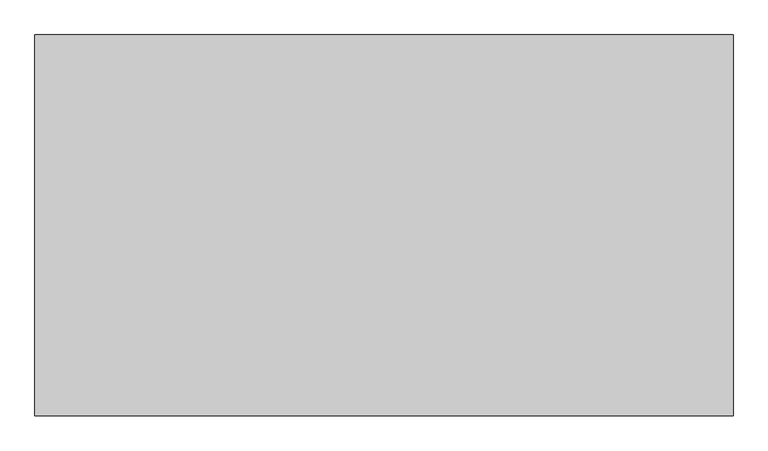
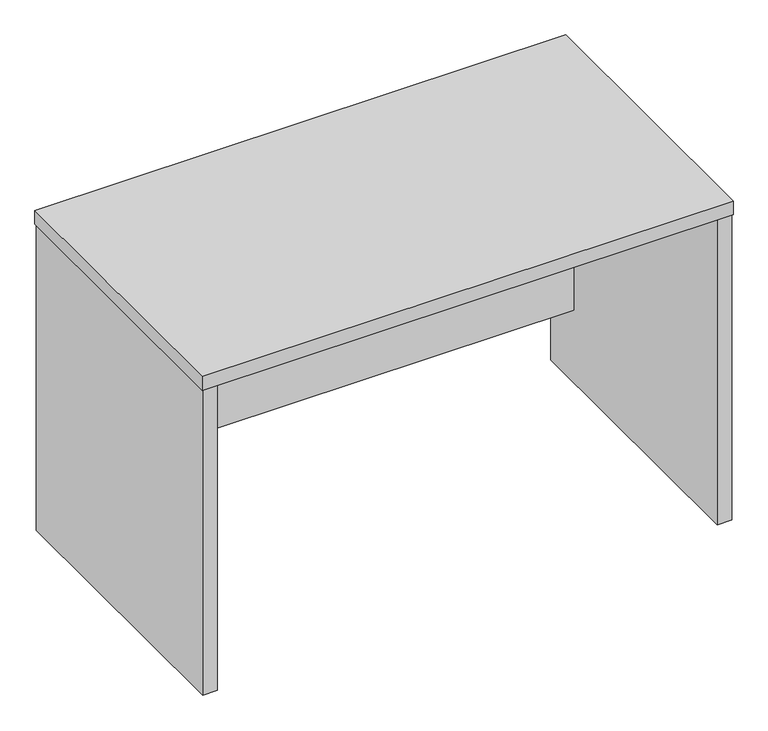
"""IFC4 building model written with IfcOpenShell, lengths in millimetres: furniture geometry, GEL-Table-一般オフィスデスク : GEL-Table-一般オフィスデスク."""

import ifcopenshell
import ifcopenshell.guid

model = None  # the IFC model being written
_history = None  # IfcOwnerHistory: only IFC2X3 demands one
_inside = {}  # id of a spatial element -> (the spatial element, [elements in it])
_under = {}  # id of a project, library or spatial element -> (it, [spatial elements below it])
_declared = {}  # id of a project -> (the project, [libraries it declares])
_typed = {}  # id of a type object -> (the type object, [elements of that type])
_made_of = {}  # id of a material, layer set ... -> (it, [elements and type objects made of it])


def new_model(schema):
    """Start an empty IFC model of exactly this schema.

    Asked for "IFC4X3", IfcOpenShell would pick the latest addendum, in which some entities
    have other attributes; the version numbers below select the first issue.
    IFC2X3 requires an IfcOwnerHistory on every rooted entity: one is made here for all.
    """
    global model, _history
    if schema == "IFC4X3":
        model = ifcopenshell.file(schema_version=(4, 3, 0, 0))
    else:
        model = ifcopenshell.file(schema=schema)
    _inside.clear()
    _under.clear()
    _declared.clear()
    _typed.clear()
    _made_of.clear()
    _history = None
    if model.schema == "IFC2X3":
        org = make("IfcOrganization", Name="unknown")
        user = make(
            "IfcPersonAndOrganization",
            ThePerson=make("IfcPerson", FamilyName="unknown"),
            TheOrganization=org,
        )
        app = make(
            "IfcApplication",
            ApplicationDeveloper=org,
            Version="unknown",
            ApplicationFullName="unknown",
            ApplicationIdentifier="unknown",
        )
        _history = make(
            "IfcOwnerHistory",
            OwningUser=user,
            OwningApplication=app,
            ChangeAction="ADDED",
            CreationDate=0,
        )
    return model


def make(cls, **values):
    """One entity of the class cls with the attributes given. An attribute that is None is left unset."""
    return model.create_entity(
        cls, **{name: value for name, value in values.items() if value is not None}
    )


def rooted(cls, **values):
    """An entity with a GlobalId (a new one), such as an element, a storey or a relation."""
    return make(cls, GlobalId=ifcopenshell.guid.new(), OwnerHistory=_history, **values)


def si_unit(unit_type, name, prefix=None):
    """IfcSIUnit, for example si_unit("LENGTHUNIT", "METRE", prefix="MILLI")."""
    return make("IfcSIUnit", UnitType=unit_type, Prefix=prefix, Name=name)


def assignment(units):
    """IfcUnitAssignment: the units of a project."""
    return None if units is None else make("IfcUnitAssignment", Units=units)


def point(xyz):
    """IfcCartesianPoint."""
    return None if xyz is None else make("IfcCartesianPoint", Coordinates=xyz)


def direction(xyz):
    """IfcDirection."""
    return None if xyz is None else make("IfcDirection", DirectionRatios=xyz)


def frame(location, z_axis=None, x_axis=None):
    """IfcAxis2Placement3D, a coordinate frame: its origin and axes. An axis left out is left unset."""
    return make(
        "IfcAxis2Placement3D",
        Location=point(location),
        Axis=direction(z_axis),
        RefDirection=direction(x_axis),
    )


def origin():
    """The frame at (0, 0, 0) with its axes left unset."""
    return frame((0.0, 0.0, 0.0))


def origin_with_axes():
    """The frame at (0, 0, 0) with the z axis (0, 0, 1) and the x axis (1, 0, 0) written out."""
    return frame((0.0, 0.0, 0.0), z_axis=(0.0, 0.0, 1.0), x_axis=(1.0, 0.0, 0.0))


def place(relative_to, where):
    """IfcLocalPlacement: puts the frame where relative to a parent placement (None: the world)."""
    return make(
        "IfcLocalPlacement", PlacementRelTo=relative_to, RelativePlacement=where
    )


def context(
    kind, dimensions, precision=None, world=None, true_north=None, identifier=None
):
    """IfcGeometricRepresentationContext, for example the 3D "Model" context."""
    return make(
        "IfcGeometricRepresentationContext",
        ContextIdentifier=identifier,
        ContextType=kind,
        CoordinateSpaceDimension=dimensions,
        Precision=precision,
        WorldCoordinateSystem=world,
        TrueNorth=true_north,
    )


def project(units=None, contexts=None):
    """IfcProject with its units and contexts."""
    return rooted(
        "IfcProject",
        Name="project",
        RepresentationContexts=contexts,
        UnitsInContext=assignment(units),
    )


def spatial(cls, under=None, at=None, **own):
    """A site, building, storey or space (cls), placed at a placement, below another one or the project."""
    s = rooted(cls, ObjectPlacement=at, **own)
    if under is not None:
        _under.setdefault(under.id(), (under, []))[1].append(s)
    return s


def polyline(points):
    """IfcPolyline through the points."""
    return make("IfcPolyline", Points=[point(p) for p in points])


def outline(outer, holes=None, kind="AREA"):
    """IfcArbitraryClosedProfileDef: a profile drawn as a closed curve; with holes, ...WithVoids."""
    if holes is None:
        return make("IfcArbitraryClosedProfileDef", ProfileType=kind, OuterCurve=outer)
    return make(
        "IfcArbitraryProfileDefWithVoids",
        ProfileType=kind,
        OuterCurve=outer,
        InnerCurves=holes,
    )


def extrude(swept, where, along, depth):
    """IfcExtrudedAreaSolid: the profile swept, set in the frame where, extruded along a direction by depth."""
    return make(
        "IfcExtrudedAreaSolid",
        SweptArea=swept,
        Position=where,
        ExtrudedDirection=direction(along),
        Depth=depth,
    )


def shape(context_of_items, identifier, shape_type, items):
    """IfcShapeRepresentation: the items that make up one representation, for example the "Body"."""
    return make(
        "IfcShapeRepresentation",
        ContextOfItems=context_of_items,
        RepresentationIdentifier=identifier,
        RepresentationType=shape_type,
        Items=items,
    )


def source(mapping_origin, context_of_items, identifier, shape_type, items):
    """IfcRepresentationMap: a shape defined once, which mapped items show again and again."""
    return make(
        "IfcRepresentationMap",
        MappingOrigin=mapping_origin,
        MappedRepresentation=shape(context_of_items, identifier, shape_type, items),
    )


def transform(
    local_origin,
    x_axis=None,
    y_axis=None,
    z_axis=None,
    scale=None,
    scale2=None,
    scale3=None,
    uniform=True,
):
    """IfcCartesianTransformationOperator3D, or its non-uniform kind. x_axis, y_axis, z_axis: its Axis1, 2, 3."""
    if uniform:
        return make(
            "IfcCartesianTransformationOperator3D",
            Axis1=direction(x_axis),
            Axis2=direction(y_axis),
            LocalOrigin=point(local_origin),
            Scale=scale,
            Axis3=direction(z_axis),
        )
    return make(
        "IfcCartesianTransformationOperator3DnonUniform",
        Axis1=direction(x_axis),
        Axis2=direction(y_axis),
        LocalOrigin=point(local_origin),
        Scale=scale,
        Axis3=direction(z_axis),
        Scale2=scale2,
        Scale3=scale3,
    )


def mapped(mapping_source, mapping_target):
    """IfcMappedItem: shows the shape of a source again, moved by a transform."""
    return make(
        "IfcMappedItem", MappingSource=mapping_source, MappingTarget=mapping_target
    )


def made_of(thing, what):
    """Note that an element or type object is made of a material, layer set ...; save() writes the relation."""
    if what is not None:
        _made_of.setdefault(what.id(), (what, []))[1].append(thing)
    return thing


def element(
    cls,
    number,
    at=None,
    inside=None,
    cuts=None,
    type_object=None,
    material=None,
    context=None,
    identifier="Body",
    shape_type=None,
    held_by="IfcProductDefinitionShape",
    body=None,
    shapes=None,
    **own,
):
    """One element of the class cls, such as IfcWall. Its Tag is "e" and its number.

    at: its placement. inside: the storey or other place that contains it. cuts: it is an
    opening in that element (IfcRelVoidsElement). A single representation is given by context,
    identifier, shape_type and body (its items); several are given by shapes. held_by: the class
    of the entity that holds the representations. save() writes the other relations.
    """
    e = rooted(cls, Tag="e%d" % number, ObjectPlacement=at, **own)
    if body is not None:
        shapes = [shape(context, identifier, shape_type, body)]
    if shapes is not None:
        e.Representation = make(held_by, Representations=shapes)
    if inside is not None:
        _inside.setdefault(inside.id(), (inside, []))[1].append(e)
    if cuts is not None:
        rooted(
            "IfcRelVoidsElement", RelatingBuildingElement=cuts, RelatedOpeningElement=e
        )
    if type_object is not None:
        _typed.setdefault(type_object.id(), (type_object, []))[1].append(e)
    return made_of(e, material)


def aggregate(whole, parts):
    """IfcRelAggregates: a whole, such as a stair, and the parts it consists of."""
    return rooted("IfcRelAggregates", RelatingObject=whole, RelatedObjects=parts)


def save(model, path):
    """Write the relations noted so far, then the file.

    IfcRelAggregates (storeys below a building ...), IfcRelContainedInSpatialStructure (elements
    in a storey), IfcRelDefinesByType, IfcRelAssociatesMaterial and IfcRelDeclares: one each for
    every whole, place, type object, material and project.
    """
    for whole, parts in _under.values():
        aggregate(whole, parts)
    for where, things in _inside.values():
        rooted(
            "IfcRelContainedInSpatialStructure",
            RelatedElements=things,
            RelatingStructure=where,
        )
    for kind, things in _typed.values():
        rooted("IfcRelDefinesByType", RelatedObjects=things, RelatingType=kind)
    for what, things in _made_of.values():
        rooted("IfcRelAssociatesMaterial", RelatedObjects=things, RelatingMaterial=what)
    for by, libraries in _declared.values():
        rooted("IfcRelDeclares", RelatingContext=by, RelatedDefinitions=libraries)
    model.write(path)


def furniture_45d6af98(model_context):
    return source(origin(), model_context, "Body", "SweptSolid", [
        extrude(outline(polyline([(-518.0, 217.0), (-518.0, 247.0), (518.0, 247.0), (518.0, 217.0), (-518.0, 217.0)])), frame((0.0, 0.0, 160.0), z_axis=(0.0, 0.0, 1.0), x_axis=(1.0, 0.0, 0.0)), (0.0, 0.0, 1.0), 510.0),
        extrude(outline(polyline([(518.0, -296.0), (518.0, 300.0), (548.0, 300.0), (548.0, -296.0), (518.0, -296.0)])), origin_with_axes(), (0.0, 0.0, 1.0), 670.0),
        extrude(outline(polyline([(-548.0, -296.0), (-548.0, 300.0), (-518.0, 300.0), (-518.0, -296.0), (-548.0, -296.0)])), origin_with_axes(), (0.0, 0.0, 1.0), 670.0),
        extrude(outline(polyline([(-550.0, -298.0), (-550.0, 302.0), (550.0, 302.0), (550.0, -298.0), (-550.0, -298.0)])), frame((0.0, 0.0, 670.0), z_axis=(0.0, 0.0, 1.0), x_axis=(1.0, 0.0, 0.0)), (0.0, 0.0, 1.0), 30.0),
    ])


if __name__ == "__main__":
    model = new_model("IFC4")
    model_context = context("Model", 3, world=origin())
    ifc_project = project(units=[si_unit("LENGTHUNIT", "METRE", prefix="MILLI")], contexts=[model_context])
    site = spatial("IfcSite", under=ifc_project)
    building = spatial("IfcBuilding", under=site)
    placement = place(None, origin())
    furniture_shape = furniture_45d6af98(model_context)
    element("IfcFurniture", 1, ObjectType="GEL-Table-一般オフィスデスク : GEL-Table-一般オフィスデスク", at=placement, inside=building, context=model_context, shape_type="MappedRepresentation", body=[
        mapped(furniture_shape, transform((0.0, 0.0, 0.0), x_axis=(1.0, 0.0, 0.0), y_axis=(0.0, 1.0, 0.0), z_axis=(0.0, 0.0, 1.0))),
    ])
    save(model, "model.ifc")

# Revit data of these elements
# Type "GEL-Table-一般オフィスデスク : GEL-Table-一般オフィスデスク"
#   GEL-Width = 1100 mm
#   GEL-Height = 700 mm
#   GEL-Depth = 600 mm
#   GEL-Material-Top = Walnut brown polished
#   GEL-Material-Support = Walnut brown polished
#   GEL-Material-Base = none
#   GEL-Material-Accent = none
#   Default Elevation = 0
# Element 1 (IfcFurniture, "GEL-Table-一般オフィスデスク : GEL-Table-一般オフィスデスク")
#   Materials on its faces: "Walnut brown polished"
# Materials
#   "Walnut brown polished": class "一般", colour RGB 103 67 45, transparency 0, Cost = 0
